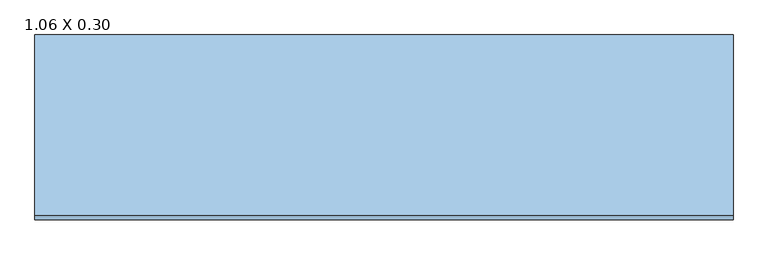
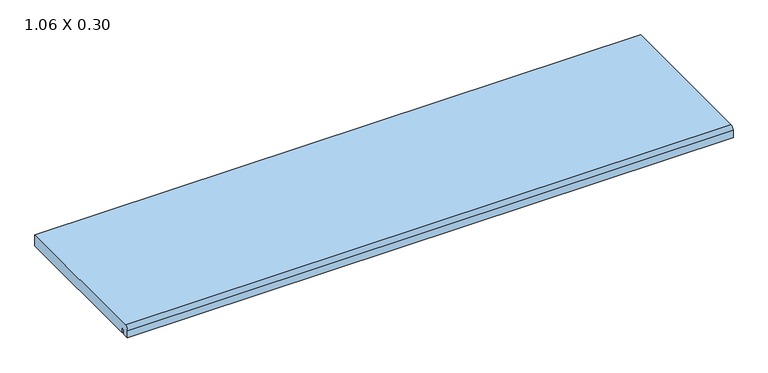
"""IFC4 building model written with IfcOpenShell, lengths in millimetres: window geometry, .CC_ND 300_PEDRA_PEITORIL RETO : 1.06 X 0.30."""

from ifc_helpers import new_model, si_unit, point, frame, frame_2d, origin, place, context, project, spatial, polyline, circle_curve, trimmed, segment, composite_curve, outline, extrude, source, transform, mapped, element, save


def window_1_06_x_0_30_ddfe798f(model_context):
    return source(origin(), model_context, "Body", "SweptSolid", [
        extrude(outline(composite_curve([segment(polyline([(-132.5083081, 1480.0), (-132.5083081, 1488.1993124), (-137.2619526, 1488.1993124), (-137.2619526, 1480.0), (-148.0, 1480.0), (-148.0, 1493.3808343)]), True, "CONTINUOUS"), segment(trimmed(circle_curve(frame_2d((-141.3808343, 1493.3808343)), 6.6191657), [point((-148.0, 1493.3808343))], [point((-141.3808343, 1500.0))], False, "CARTESIAN"), True, "CONTINUOUS"), segment(polyline([(-141.3808343, 1500.0), (132.7, 1500.0), (132.7, 1480.0), (-132.5083081, 1480.0)]), True, "CONTINUOUS")], self_intersect=False)), frame((-530.0, 0.0, 0.0), z_axis=(1.0, 0.0, 0.0), x_axis=(0.0, 1.0, 0.0)), (0.0, 0.0, 1.0), 1060.0),
    ])


if __name__ == "__main__":
    model = new_model("IFC4")
    model_context = context("Model", 3, world=origin())
    ifc_project = project(units=[si_unit("LENGTHUNIT", "METRE", prefix="MILLI")], contexts=[model_context])
    site = spatial("IfcSite", under=ifc_project)
    building = spatial("IfcBuilding", under=site)
    placement = place(None, origin())
    window_1_06_x_0_30_shape = window_1_06_x_0_30_ddfe798f(model_context)
    element("IfcWindow", 1, ObjectType=".CC_ND 300_PEDRA_PEITORIL RETO : 1.06 X 0.30", at=placement, inside=building, context=model_context, shape_type="MappedRepresentation", body=[
        mapped(window_1_06_x_0_30_shape, transform((0.0, 0.0, 0.0), x_axis=(1.0, 0.0, 0.0), y_axis=(0.0, 1.0, 0.0), z_axis=(0.0, 0.0, 1.0))),
    ])
    save(model, "model.ifc")

# Revit data of these elements
# Type ".CC_ND 300_PEDRA_PEITORIL RETO : 1.06 X 0.30"
#   Type Mark = "68"
#   Largura da pedra [instance default] = 0.26 m
#   Extensão interior peitoril [instance default] = 0.03 m
#   Extensão exterior peitoril [instance default] = 0.03 m
#   Espessura = 0.02 m
#   Comprimento = 1.06 m
#   Altura-padrão do peitoril = 1.48 m
#   Peitoril = .GRANITO_BRANCO_ITAUNAS
#   Rough Width = 0
#   Rough Height = 0
#   Height = 0
#   Wall Closure = (empty or 0)
#   Width = 0
# Element 1 (IfcWindow, ".CC_ND 300_PEDRA_PEITORIL RETO : 1.06 X 0.30")
#   Largura da pedra = 0.2807 m
#   Extensão interior peitoril = 0.0147 m
#   Materials on its faces: ".GRANITO_BRANCO_ITAUNAS"
# Materials
#   ".GRANITO_BRANCO_ITAUNAS": class ".CC_PEDRA REVEST.", colour RGB 202 195 174, transparency 0, Description = "Revestimento em granito", Cost = 0
